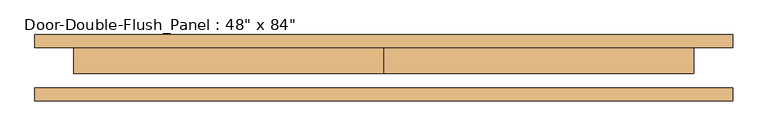
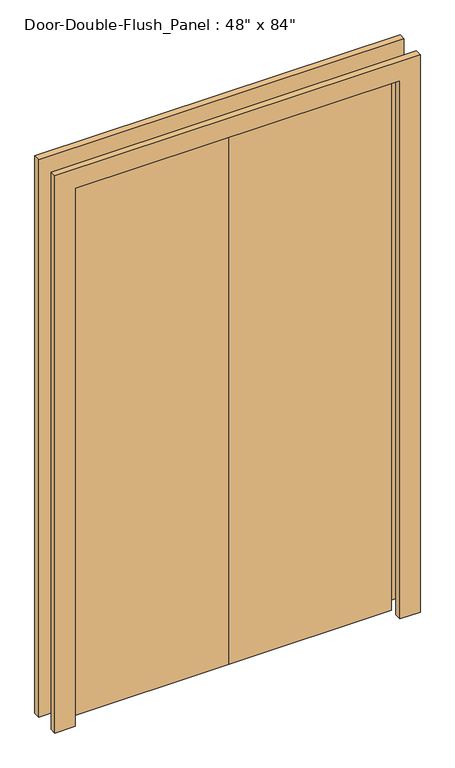
"""IFC4 building model written with IfcOpenShell, lengths in millimetres: door geometry."""

import ifcopenshell
import ifcopenshell.guid

model = None  # the IFC model being written
_history = None  # IfcOwnerHistory: only IFC2X3 demands one
_inside = {}  # id of a spatial element -> (the spatial element, [elements in it])
_under = {}  # id of a project, library or spatial element -> (it, [spatial elements below it])
_declared = {}  # id of a project -> (the project, [libraries it declares])
_typed = {}  # id of a type object -> (the type object, [elements of that type])
_made_of = {}  # id of a material, layer set ... -> (it, [elements and type objects made of it])


def new_model(schema):
    """Start an empty IFC model of exactly this schema.

    Asked for "IFC4X3", IfcOpenShell would pick the latest addendum, in which some entities
    have other attributes; the version numbers below select the first issue.
    IFC2X3 requires an IfcOwnerHistory on every rooted entity: one is made here for all.
    """
    global model, _history
    if schema == "IFC4X3":
        model = ifcopenshell.file(schema_version=(4, 3, 0, 0))
    else:
        model = ifcopenshell.file(schema=schema)
    _inside.clear()
    _under.clear()
    _declared.clear()
    _typed.clear()
    _made_of.clear()
    _history = None
    if model.schema == "IFC2X3":
        org = make("IfcOrganization", Name="unknown")
        user = make(
            "IfcPersonAndOrganization",
            ThePerson=make("IfcPerson", FamilyName="unknown"),
            TheOrganization=org,
        )
        app = make(
            "IfcApplication",
            ApplicationDeveloper=org,
            Version="unknown",
            ApplicationFullName="unknown",
            ApplicationIdentifier="unknown",
        )
        _history = make(
            "IfcOwnerHistory",
            OwningUser=user,
            OwningApplication=app,
            ChangeAction="ADDED",
            CreationDate=0,
        )
    return model


def make(cls, **values):
    """One entity of the class cls with the attributes given. An attribute that is None is left unset."""
    return model.create_entity(
        cls, **{name: value for name, value in values.items() if value is not None}
    )


def rooted(cls, **values):
    """An entity with a GlobalId (a new one), such as an element, a storey or a relation."""
    return make(cls, GlobalId=ifcopenshell.guid.new(), OwnerHistory=_history, **values)


def si_unit(unit_type, name, prefix=None):
    """IfcSIUnit, for example si_unit("LENGTHUNIT", "METRE", prefix="MILLI")."""
    return make("IfcSIUnit", UnitType=unit_type, Prefix=prefix, Name=name)


def assignment(units):
    """IfcUnitAssignment: the units of a project."""
    return None if units is None else make("IfcUnitAssignment", Units=units)


def point(xyz):
    """IfcCartesianPoint."""
    return None if xyz is None else make("IfcCartesianPoint", Coordinates=xyz)


def direction(xyz):
    """IfcDirection."""
    return None if xyz is None else make("IfcDirection", DirectionRatios=xyz)


def frame(location, z_axis=None, x_axis=None):
    """IfcAxis2Placement3D, a coordinate frame: its origin and axes. An axis left out is left unset."""
    return make(
        "IfcAxis2Placement3D",
        Location=point(location),
        Axis=direction(z_axis),
        RefDirection=direction(x_axis),
    )


def origin():
    """The frame at (0, 0, 0) with its axes left unset."""
    return frame((0.0, 0.0, 0.0))


def origin_with_axes():
    """The frame at (0, 0, 0) with the z axis (0, 0, 1) and the x axis (1, 0, 0) written out."""
    return frame((0.0, 0.0, 0.0), z_axis=(0.0, 0.0, 1.0), x_axis=(1.0, 0.0, 0.0))


def place(relative_to, where):
    """IfcLocalPlacement: puts the frame where relative to a parent placement (None: the world)."""
    return make(
        "IfcLocalPlacement", PlacementRelTo=relative_to, RelativePlacement=where
    )


def context(
    kind, dimensions, precision=None, world=None, true_north=None, identifier=None
):
    """IfcGeometricRepresentationContext, for example the 3D "Model" context."""
    return make(
        "IfcGeometricRepresentationContext",
        ContextIdentifier=identifier,
        ContextType=kind,
        CoordinateSpaceDimension=dimensions,
        Precision=precision,
        WorldCoordinateSystem=world,
        TrueNorth=true_north,
    )


def project(units=None, contexts=None):
    """IfcProject with its units and contexts."""
    return rooted(
        "IfcProject",
        Name="project",
        RepresentationContexts=contexts,
        UnitsInContext=assignment(units),
    )


def spatial(cls, under=None, at=None, **own):
    """A site, building, storey or space (cls), placed at a placement, below another one or the project."""
    s = rooted(cls, ObjectPlacement=at, **own)
    if under is not None:
        _under.setdefault(under.id(), (under, []))[1].append(s)
    return s


def polyline(points):
    """IfcPolyline through the points."""
    return make("IfcPolyline", Points=[point(p) for p in points])


def outline(outer, holes=None, kind="AREA"):
    """IfcArbitraryClosedProfileDef: a profile drawn as a closed curve; with holes, ...WithVoids."""
    if holes is None:
        return make("IfcArbitraryClosedProfileDef", ProfileType=kind, OuterCurve=outer)
    return make(
        "IfcArbitraryProfileDefWithVoids",
        ProfileType=kind,
        OuterCurve=outer,
        InnerCurves=holes,
    )


def extrude(swept, where, along, depth):
    """IfcExtrudedAreaSolid: the profile swept, set in the frame where, extruded along a direction by depth."""
    return make(
        "IfcExtrudedAreaSolid",
        SweptArea=swept,
        Position=where,
        ExtrudedDirection=direction(along),
        Depth=depth,
    )


def shape(context_of_items, identifier, shape_type, items):
    """IfcShapeRepresentation: the items that make up one representation, for example the "Body"."""
    return make(
        "IfcShapeRepresentation",
        ContextOfItems=context_of_items,
        RepresentationIdentifier=identifier,
        RepresentationType=shape_type,
        Items=items,
    )


def source(mapping_origin, context_of_items, identifier, shape_type, items):
    """IfcRepresentationMap: a shape defined once, which mapped items show again and again."""
    return make(
        "IfcRepresentationMap",
        MappingOrigin=mapping_origin,
        MappedRepresentation=shape(context_of_items, identifier, shape_type, items),
    )


def transform(
    local_origin,
    x_axis=None,
    y_axis=None,
    z_axis=None,
    scale=None,
    scale2=None,
    scale3=None,
    uniform=True,
):
    """IfcCartesianTransformationOperator3D, or its non-uniform kind. x_axis, y_axis, z_axis: its Axis1, 2, 3."""
    if uniform:
        return make(
            "IfcCartesianTransformationOperator3D",
            Axis1=direction(x_axis),
            Axis2=direction(y_axis),
            LocalOrigin=point(local_origin),
            Scale=scale,
            Axis3=direction(z_axis),
        )
    return make(
        "IfcCartesianTransformationOperator3DnonUniform",
        Axis1=direction(x_axis),
        Axis2=direction(y_axis),
        LocalOrigin=point(local_origin),
        Scale=scale,
        Axis3=direction(z_axis),
        Scale2=scale2,
        Scale3=scale3,
    )


def mapped(mapping_source, mapping_target):
    """IfcMappedItem: shows the shape of a source again, moved by a transform."""
    return make(
        "IfcMappedItem", MappingSource=mapping_source, MappingTarget=mapping_target
    )


def made_of(thing, what):
    """Note that an element or type object is made of a material, layer set ...; save() writes the relation."""
    if what is not None:
        _made_of.setdefault(what.id(), (what, []))[1].append(thing)
    return thing


def element(
    cls,
    number,
    at=None,
    inside=None,
    cuts=None,
    type_object=None,
    material=None,
    context=None,
    identifier="Body",
    shape_type=None,
    held_by="IfcProductDefinitionShape",
    body=None,
    shapes=None,
    **own,
):
    """One element of the class cls, such as IfcWall. Its Tag is "e" and its number.

    at: its placement. inside: the storey or other place that contains it. cuts: it is an
    opening in that element (IfcRelVoidsElement). A single representation is given by context,
    identifier, shape_type and body (its items); several are given by shapes. held_by: the class
    of the entity that holds the representations. save() writes the other relations.
    """
    e = rooted(cls, Tag="e%d" % number, ObjectPlacement=at, **own)
    if body is not None:
        shapes = [shape(context, identifier, shape_type, body)]
    if shapes is not None:
        e.Representation = make(held_by, Representations=shapes)
    if inside is not None:
        _inside.setdefault(inside.id(), (inside, []))[1].append(e)
    if cuts is not None:
        rooted(
            "IfcRelVoidsElement", RelatingBuildingElement=cuts, RelatedOpeningElement=e
        )
    if type_object is not None:
        _typed.setdefault(type_object.id(), (type_object, []))[1].append(e)
    return made_of(e, material)


def aggregate(whole, parts):
    """IfcRelAggregates: a whole, such as a stair, and the parts it consists of."""
    return rooted("IfcRelAggregates", RelatingObject=whole, RelatedObjects=parts)


def save(model, path):
    """Write the relations noted so far, then the file.

    IfcRelAggregates (storeys below a building ...), IfcRelContainedInSpatialStructure (elements
    in a storey), IfcRelDefinesByType, IfcRelAssociatesMaterial and IfcRelDeclares: one each for
    every whole, place, type object, material and project.
    """
    for whole, parts in _under.values():
        aggregate(whole, parts)
    for where, things in _inside.values():
        rooted(
            "IfcRelContainedInSpatialStructure",
            RelatedElements=things,
            RelatingStructure=where,
        )
    for kind, things in _typed.values():
        rooted("IfcRelDefinesByType", RelatedObjects=things, RelatingType=kind)
    for what, things in _made_of.values():
        rooted("IfcRelAssociatesMaterial", RelatedObjects=things, RelatingMaterial=what)
    for by, libraries in _declared.values():
        rooted("IfcRelDeclares", RelatingContext=by, RelatedDefinitions=libraries)
    model.write(path)


def door_f69827bf(model_context):
    return source(origin(), model_context, "Body", "SweptSolid", [
        extrude(outline(polyline([(2133.6, -609.6), (2133.6, 609.6), (0.0, 609.6), (0.0, 685.8), (2209.8, 685.8), (2209.8, -685.8), (0.0, -685.8), (0.0, -609.6), (2133.6, -609.6)])), frame((0.0, -65.0875, 0.0), z_axis=(0.0, 1.0, 0.0), x_axis=(0.0, 0.0, 1.0)), (0.0, 0.0, 1.0), 25.4),
        extrude(outline(polyline([(2133.6, -609.6), (2133.6, 609.6), (0.0, 609.6), (0.0, 685.8), (2209.8, 685.8), (2209.8, -685.8), (0.0, -685.8), (0.0, -609.6), (2133.6, -609.6)])), frame((0.0, 39.6875, 0.0), z_axis=(0.0, 1.0, 0.0), x_axis=(0.0, 0.0, 1.0)), (0.0, 0.0, 1.0), 25.4),
        extrude(outline(polyline([(0.0, 39.6875), (609.6, 39.6875), (609.6, -11.1125), (0.0, -11.1125), (0.0, 39.6875)])), origin_with_axes(), (0.0, 0.0, 1.0), 2133.6),
        extrude(outline(polyline([(-609.6, 39.6875), (0.0, 39.6875), (0.0, -11.1125), (-609.6, -11.1125), (-609.6, 39.6875)])), origin_with_axes(), (0.0, 0.0, 1.0), 2133.6),
    ])


if __name__ == "__main__":
    model = new_model("IFC4")
    model_context = context("Model", 3, world=origin())
    ifc_project = project(units=[si_unit("LENGTHUNIT", "METRE", prefix="MILLI")], contexts=[model_context])
    site = spatial("IfcSite", under=ifc_project)
    building = spatial("IfcBuilding", under=site)
    placement = place(None, origin())
    door_shape = door_f69827bf(model_context)
    element("IfcDoor", 1, ObjectType="Door-Double-Flush_Panel : 48\" x 84\"", at=placement, inside=building, context=model_context, shape_type="MappedRepresentation", body=[
        mapped(door_shape, transform((0.0, 0.0, 0.0), x_axis=(1.0, 0.0, 0.0), y_axis=(0.0, 1.0, 0.0), z_axis=(0.0, 0.0, 1.0))),
    ])
    save(model, "model.ifc")

# Revit data of these elements
# Type "Door-Double-Flush_Panel : 48\" x 84\""
#   Type Mark = "8"
#   Fire Rating = "60 Mins"
#   Construction Type Id = "DOOR"
#   Assembly Code = "C1020"
#   Analytic Construction = "Wooden"
#   Thickness = 0' - 2"
#   Thermal Resistance (R) = 2.5876 (h·ft²·°F)/BTU
#   Swing Angle [instance default] = 90.00°
#   Panel Width = 2' - 0"
#   Heat Transfer Coefficient (U) = 0.3865 BTU/(h·ft²·°F)
#   Height = 7' - 0"
#   Trim Projection Ext = 0' - 1"
#   Trim Projection Int = 0' - 1"
#   Trim Width = 0' - 3"
#   Width = 4' - 0"
#   Define Thermal Properties by = 1
#   Panel Material = Wood - Birch - Solid Stained Light Low Gloss
#   Trim Material = Paint - Sienna
#   Visual Light Transmittance = 0
#   Solar Heat Gain Coefficient = 0
#   Function = (empty or 0)
#   Wall Closure = (empty or 0)
# Element 1 (IfcDoor, "Door-Double-Flush_Panel : 48\" x 84\"")
#   Materials on its faces: "Paint - Sienna", "Wood - Birch - Solid Stained Light Low Gloss"
# Materials
#   "Wood - Birch - Solid Stained Light Low Gloss": class "Wood", colour RGB 210 159 95, transparency 0, Cost = 0
#   "Paint - Sienna": class "Miscellaneous", colour RGB 118 70 51, transparency 0, Cost = 0
